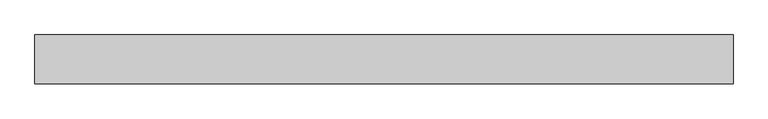
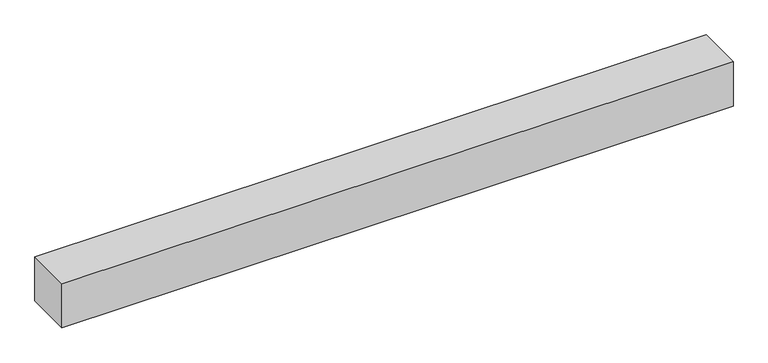
"""IFC4 building model written with IfcOpenShell, lengths in millimetres: proxy geometry, Structure019 936 : Structure019 936."""

import ifcopenshell
import ifcopenshell.guid

model = None  # the IFC model being written
_history = None  # IfcOwnerHistory: only IFC2X3 demands one
_inside = {}  # id of a spatial element -> (the spatial element, [elements in it])
_under = {}  # id of a project, library or spatial element -> (it, [spatial elements below it])
_declared = {}  # id of a project -> (the project, [libraries it declares])
_typed = {}  # id of a type object -> (the type object, [elements of that type])
_made_of = {}  # id of a material, layer set ... -> (it, [elements and type objects made of it])


def new_model(schema):
    """Start an empty IFC model of exactly this schema.

    Asked for "IFC4X3", IfcOpenShell would pick the latest addendum, in which some entities
    have other attributes; the version numbers below select the first issue.
    IFC2X3 requires an IfcOwnerHistory on every rooted entity: one is made here for all.
    """
    global model, _history
    if schema == "IFC4X3":
        model = ifcopenshell.file(schema_version=(4, 3, 0, 0))
    else:
        model = ifcopenshell.file(schema=schema)
    _inside.clear()
    _under.clear()
    _declared.clear()
    _typed.clear()
    _made_of.clear()
    _history = None
    if model.schema == "IFC2X3":
        org = make("IfcOrganization", Name="unknown")
        user = make(
            "IfcPersonAndOrganization",
            ThePerson=make("IfcPerson", FamilyName="unknown"),
            TheOrganization=org,
        )
        app = make(
            "IfcApplication",
            ApplicationDeveloper=org,
            Version="unknown",
            ApplicationFullName="unknown",
            ApplicationIdentifier="unknown",
        )
        _history = make(
            "IfcOwnerHistory",
            OwningUser=user,
            OwningApplication=app,
            ChangeAction="ADDED",
            CreationDate=0,
        )
    return model


def make(cls, **values):
    """One entity of the class cls with the attributes given. An attribute that is None is left unset."""
    return model.create_entity(
        cls, **{name: value for name, value in values.items() if value is not None}
    )


def rooted(cls, **values):
    """An entity with a GlobalId (a new one), such as an element, a storey or a relation."""
    return make(cls, GlobalId=ifcopenshell.guid.new(), OwnerHistory=_history, **values)


def si_unit(unit_type, name, prefix=None):
    """IfcSIUnit, for example si_unit("LENGTHUNIT", "METRE", prefix="MILLI")."""
    return make("IfcSIUnit", UnitType=unit_type, Prefix=prefix, Name=name)


def assignment(units):
    """IfcUnitAssignment: the units of a project."""
    return None if units is None else make("IfcUnitAssignment", Units=units)


def point(xyz):
    """IfcCartesianPoint."""
    return None if xyz is None else make("IfcCartesianPoint", Coordinates=xyz)


def direction(xyz):
    """IfcDirection."""
    return None if xyz is None else make("IfcDirection", DirectionRatios=xyz)


def frame(location, z_axis=None, x_axis=None):
    """IfcAxis2Placement3D, a coordinate frame: its origin and axes. An axis left out is left unset."""
    return make(
        "IfcAxis2Placement3D",
        Location=point(location),
        Axis=direction(z_axis),
        RefDirection=direction(x_axis),
    )


def origin():
    """The frame at (0, 0, 0) with its axes left unset."""
    return frame((0.0, 0.0, 0.0))


def place(relative_to, where):
    """IfcLocalPlacement: puts the frame where relative to a parent placement (None: the world)."""
    return make(
        "IfcLocalPlacement", PlacementRelTo=relative_to, RelativePlacement=where
    )


def context(
    kind, dimensions, precision=None, world=None, true_north=None, identifier=None
):
    """IfcGeometricRepresentationContext, for example the 3D "Model" context."""
    return make(
        "IfcGeometricRepresentationContext",
        ContextIdentifier=identifier,
        ContextType=kind,
        CoordinateSpaceDimension=dimensions,
        Precision=precision,
        WorldCoordinateSystem=world,
        TrueNorth=true_north,
    )


def project(units=None, contexts=None):
    """IfcProject with its units and contexts."""
    return rooted(
        "IfcProject",
        Name="project",
        RepresentationContexts=contexts,
        UnitsInContext=assignment(units),
    )


def spatial(cls, under=None, at=None, **own):
    """A site, building, storey or space (cls), placed at a placement, below another one or the project."""
    s = rooted(cls, ObjectPlacement=at, **own)
    if under is not None:
        _under.setdefault(under.id(), (under, []))[1].append(s)
    return s


def polyline(points):
    """IfcPolyline through the points."""
    return make("IfcPolyline", Points=[point(p) for p in points])


def outline(outer, holes=None, kind="AREA"):
    """IfcArbitraryClosedProfileDef: a profile drawn as a closed curve; with holes, ...WithVoids."""
    if holes is None:
        return make("IfcArbitraryClosedProfileDef", ProfileType=kind, OuterCurve=outer)
    return make(
        "IfcArbitraryProfileDefWithVoids",
        ProfileType=kind,
        OuterCurve=outer,
        InnerCurves=holes,
    )


def extrude(swept, where, along, depth):
    """IfcExtrudedAreaSolid: the profile swept, set in the frame where, extruded along a direction by depth."""
    return make(
        "IfcExtrudedAreaSolid",
        SweptArea=swept,
        Position=where,
        ExtrudedDirection=direction(along),
        Depth=depth,
    )


def shape(context_of_items, identifier, shape_type, items):
    """IfcShapeRepresentation: the items that make up one representation, for example the "Body"."""
    return make(
        "IfcShapeRepresentation",
        ContextOfItems=context_of_items,
        RepresentationIdentifier=identifier,
        RepresentationType=shape_type,
        Items=items,
    )


def source(mapping_origin, context_of_items, identifier, shape_type, items):
    """IfcRepresentationMap: a shape defined once, which mapped items show again and again."""
    return make(
        "IfcRepresentationMap",
        MappingOrigin=mapping_origin,
        MappedRepresentation=shape(context_of_items, identifier, shape_type, items),
    )


def transform(
    local_origin,
    x_axis=None,
    y_axis=None,
    z_axis=None,
    scale=None,
    scale2=None,
    scale3=None,
    uniform=True,
):
    """IfcCartesianTransformationOperator3D, or its non-uniform kind. x_axis, y_axis, z_axis: its Axis1, 2, 3."""
    if uniform:
        return make(
            "IfcCartesianTransformationOperator3D",
            Axis1=direction(x_axis),
            Axis2=direction(y_axis),
            LocalOrigin=point(local_origin),
            Scale=scale,
            Axis3=direction(z_axis),
        )
    return make(
        "IfcCartesianTransformationOperator3DnonUniform",
        Axis1=direction(x_axis),
        Axis2=direction(y_axis),
        LocalOrigin=point(local_origin),
        Scale=scale,
        Axis3=direction(z_axis),
        Scale2=scale2,
        Scale3=scale3,
    )


def mapped(mapping_source, mapping_target):
    """IfcMappedItem: shows the shape of a source again, moved by a transform."""
    return make(
        "IfcMappedItem", MappingSource=mapping_source, MappingTarget=mapping_target
    )


def made_of(thing, what):
    """Note that an element or type object is made of a material, layer set ...; save() writes the relation."""
    if what is not None:
        _made_of.setdefault(what.id(), (what, []))[1].append(thing)
    return thing


def element(
    cls,
    number,
    at=None,
    inside=None,
    cuts=None,
    type_object=None,
    material=None,
    context=None,
    identifier="Body",
    shape_type=None,
    held_by="IfcProductDefinitionShape",
    body=None,
    shapes=None,
    **own,
):
    """One element of the class cls, such as IfcWall. Its Tag is "e" and its number.

    at: its placement. inside: the storey or other place that contains it. cuts: it is an
    opening in that element (IfcRelVoidsElement). A single representation is given by context,
    identifier, shape_type and body (its items); several are given by shapes. held_by: the class
    of the entity that holds the representations. save() writes the other relations.
    """
    e = rooted(cls, Tag="e%d" % number, ObjectPlacement=at, **own)
    if body is not None:
        shapes = [shape(context, identifier, shape_type, body)]
    if shapes is not None:
        e.Representation = make(held_by, Representations=shapes)
    if inside is not None:
        _inside.setdefault(inside.id(), (inside, []))[1].append(e)
    if cuts is not None:
        rooted(
            "IfcRelVoidsElement", RelatingBuildingElement=cuts, RelatedOpeningElement=e
        )
    if type_object is not None:
        _typed.setdefault(type_object.id(), (type_object, []))[1].append(e)
    return made_of(e, material)


def aggregate(whole, parts):
    """IfcRelAggregates: a whole, such as a stair, and the parts it consists of."""
    return rooted("IfcRelAggregates", RelatingObject=whole, RelatedObjects=parts)


def save(model, path):
    """Write the relations noted so far, then the file.

    IfcRelAggregates (storeys below a building ...), IfcRelContainedInSpatialStructure (elements
    in a storey), IfcRelDefinesByType, IfcRelAssociatesMaterial and IfcRelDeclares: one each for
    every whole, place, type object, material and project.
    """
    for whole, parts in _under.values():
        aggregate(whole, parts)
    for where, things in _inside.values():
        rooted(
            "IfcRelContainedInSpatialStructure",
            RelatedElements=things,
            RelatingStructure=where,
        )
    for kind, things in _typed.values():
        rooted("IfcRelDefinesByType", RelatedObjects=things, RelatingType=kind)
    for what, things in _made_of.values():
        rooted("IfcRelAssociatesMaterial", RelatedObjects=things, RelatingMaterial=what)
    for by, libraries in _declared.values():
        rooted("IfcRelDeclares", RelatingContext=by, RelatedDefinitions=libraries)
    model.write(path)


def generic_models_121e7585(model_context):
    return source(origin(), model_context, "Body", "SweptSolid", [
        extrude(outline(polyline([(3694.2883192, 10278.0250834), (3694.2883192, 10417.7250834), (5694.2883192, 10417.7250834), (5694.2883192, 10278.0250834), (3694.2883192, 10278.0250834)])), frame((0.0, 0.0, 42906.696), z_axis=(0.0, 0.0, 1.0), x_axis=(1.0, 0.0, 0.0)), (0.0, 0.0, 1.0), 139.7),
    ])


if __name__ == "__main__":
    model = new_model("IFC4")
    model_context = context("Model", 3, world=origin())
    ifc_project = project(units=[si_unit("LENGTHUNIT", "METRE", prefix="MILLI")], contexts=[model_context])
    site = spatial("IfcSite", under=ifc_project)
    building = spatial("IfcBuilding", under=site)
    placement = place(None, origin())
    generic_models_shape = generic_models_121e7585(model_context)
    element("IfcBuildingElementProxy", 1, Name="Structure019 936 : Structure019 936", ObjectType="Structure019 936 : Structure019 936", at=placement, inside=building, context=model_context, shape_type="MappedRepresentation", body=[
        mapped(generic_models_shape, transform((0.0, 0.0, 0.0), x_axis=(1.0, 0.0, 0.0), y_axis=(0.0, 1.0, 0.0), z_axis=(0.0, 0.0, 1.0))),
    ])
    save(model, "model.ifc")

# Revit data of these elements
# Type "Structure019 936 : Structure019 936"
#   NameOverride = "Structure019"
# Element 1 (IfcBuildingElementProxy, "Structure019 936 : Structure019 936")
#   Materials on its faces: "STRUCTURAL MEMBER (SEE DWGS)"
# Materials
#   "STRUCTURAL MEMBER (SEE DWGS)": class "Unassigned", colour RGB 214 178 158, transparency 0, Cost = 0
